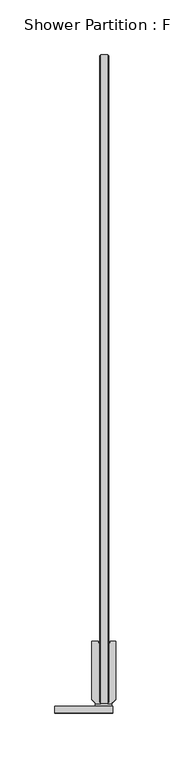
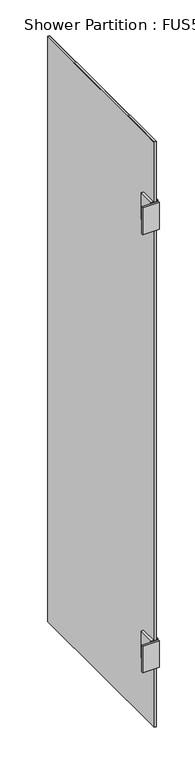
"""IFC4 building model written with IfcOpenShell, lengths in millimetres: furniture geometry, Shower Partition : FUS501_Shower Partition."""

import ifcopenshell
import ifcopenshell.guid

model = None  # the IFC model being written
_history = None  # IfcOwnerHistory: only IFC2X3 demands one
_inside = {}  # id of a spatial element -> (the spatial element, [elements in it])
_under = {}  # id of a project, library or spatial element -> (it, [spatial elements below it])
_declared = {}  # id of a project -> (the project, [libraries it declares])
_typed = {}  # id of a type object -> (the type object, [elements of that type])
_made_of = {}  # id of a material, layer set ... -> (it, [elements and type objects made of it])


def new_model(schema):
    """Start an empty IFC model of exactly this schema.

    Asked for "IFC4X3", IfcOpenShell would pick the latest addendum, in which some entities
    have other attributes; the version numbers below select the first issue.
    IFC2X3 requires an IfcOwnerHistory on every rooted entity: one is made here for all.
    """
    global model, _history
    if schema == "IFC4X3":
        model = ifcopenshell.file(schema_version=(4, 3, 0, 0))
    else:
        model = ifcopenshell.file(schema=schema)
    _inside.clear()
    _under.clear()
    _declared.clear()
    _typed.clear()
    _made_of.clear()
    _history = None
    if model.schema == "IFC2X3":
        org = make("IfcOrganization", Name="unknown")
        user = make(
            "IfcPersonAndOrganization",
            ThePerson=make("IfcPerson", FamilyName="unknown"),
            TheOrganization=org,
        )
        app = make(
            "IfcApplication",
            ApplicationDeveloper=org,
            Version="unknown",
            ApplicationFullName="unknown",
            ApplicationIdentifier="unknown",
        )
        _history = make(
            "IfcOwnerHistory",
            OwningUser=user,
            OwningApplication=app,
            ChangeAction="ADDED",
            CreationDate=0,
        )
    return model


def make(cls, **values):
    """One entity of the class cls with the attributes given. An attribute that is None is left unset."""
    return model.create_entity(
        cls, **{name: value for name, value in values.items() if value is not None}
    )


def rooted(cls, **values):
    """An entity with a GlobalId (a new one), such as an element, a storey or a relation."""
    return make(cls, GlobalId=ifcopenshell.guid.new(), OwnerHistory=_history, **values)


def si_unit(unit_type, name, prefix=None):
    """IfcSIUnit, for example si_unit("LENGTHUNIT", "METRE", prefix="MILLI")."""
    return make("IfcSIUnit", UnitType=unit_type, Prefix=prefix, Name=name)


def assignment(units):
    """IfcUnitAssignment: the units of a project."""
    return None if units is None else make("IfcUnitAssignment", Units=units)


def point(xyz):
    """IfcCartesianPoint."""
    return None if xyz is None else make("IfcCartesianPoint", Coordinates=xyz)


def direction(xyz):
    """IfcDirection."""
    return None if xyz is None else make("IfcDirection", DirectionRatios=xyz)


def frame(location, z_axis=None, x_axis=None):
    """IfcAxis2Placement3D, a coordinate frame: its origin and axes. An axis left out is left unset."""
    return make(
        "IfcAxis2Placement3D",
        Location=point(location),
        Axis=direction(z_axis),
        RefDirection=direction(x_axis),
    )


def origin():
    """The frame at (0, 0, 0) with its axes left unset."""
    return frame((0.0, 0.0, 0.0))


def place(relative_to, where):
    """IfcLocalPlacement: puts the frame where relative to a parent placement (None: the world)."""
    return make(
        "IfcLocalPlacement", PlacementRelTo=relative_to, RelativePlacement=where
    )


def context(
    kind, dimensions, precision=None, world=None, true_north=None, identifier=None
):
    """IfcGeometricRepresentationContext, for example the 3D "Model" context."""
    return make(
        "IfcGeometricRepresentationContext",
        ContextIdentifier=identifier,
        ContextType=kind,
        CoordinateSpaceDimension=dimensions,
        Precision=precision,
        WorldCoordinateSystem=world,
        TrueNorth=true_north,
    )


def project(units=None, contexts=None):
    """IfcProject with its units and contexts."""
    return rooted(
        "IfcProject",
        Name="project",
        RepresentationContexts=contexts,
        UnitsInContext=assignment(units),
    )


def spatial(cls, under=None, at=None, **own):
    """A site, building, storey or space (cls), placed at a placement, below another one or the project."""
    s = rooted(cls, ObjectPlacement=at, **own)
    if under is not None:
        _under.setdefault(under.id(), (under, []))[1].append(s)
    return s


def faces_of(points, faces, orient=None, outer=None):
    """IfcFace entities. A face is a list of loops; a loop is a list of indices into points, from 0.

    orient and outer hold one flag for each loop. By default every Orientation is true, the
    first loop of a face is its IfcFaceOuterBound and the others are IfcFaceBound.
    """
    made = []
    for i, loops in enumerate(faces):
        bounds = []
        for j, loop in enumerate(loops):
            is_outer = j == 0 if outer is None else outer[i][j]
            bounds.append(
                make(
                    "IfcFaceOuterBound" if is_outer else "IfcFaceBound",
                    Bound=make("IfcPolyLoop", Polygon=[points[k] for k in loop]),
                    Orientation=True if orient is None else orient[i][j],
                )
            )
        made.append(make("IfcFace", Bounds=bounds))
    return made


def faceted_brep(points, faces, orient=None, outer=None, voids=None):
    """IfcFacetedBrep: a solid bounded by flat faces; with voids (closed shells), ...WithVoids."""
    shared = [point(p) for p in points]
    hull = make("IfcClosedShell", CfsFaces=faces_of(shared, faces, orient, outer))
    if voids is None:
        return make("IfcFacetedBrep", Outer=hull)
    return make(
        "IfcFacetedBrepWithVoids",
        Outer=hull,
        Voids=[
            make(cls, CfsFaces=faces_of(shared, fs, o, b)) for cls, fs, o, b in voids
        ],
    )


def shape(context_of_items, identifier, shape_type, items):
    """IfcShapeRepresentation: the items that make up one representation, for example the "Body"."""
    return make(
        "IfcShapeRepresentation",
        ContextOfItems=context_of_items,
        RepresentationIdentifier=identifier,
        RepresentationType=shape_type,
        Items=items,
    )


def source(mapping_origin, context_of_items, identifier, shape_type, items):
    """IfcRepresentationMap: a shape defined once, which mapped items show again and again."""
    return make(
        "IfcRepresentationMap",
        MappingOrigin=mapping_origin,
        MappedRepresentation=shape(context_of_items, identifier, shape_type, items),
    )


def transform(
    local_origin,
    x_axis=None,
    y_axis=None,
    z_axis=None,
    scale=None,
    scale2=None,
    scale3=None,
    uniform=True,
):
    """IfcCartesianTransformationOperator3D, or its non-uniform kind. x_axis, y_axis, z_axis: its Axis1, 2, 3."""
    if uniform:
        return make(
            "IfcCartesianTransformationOperator3D",
            Axis1=direction(x_axis),
            Axis2=direction(y_axis),
            LocalOrigin=point(local_origin),
            Scale=scale,
            Axis3=direction(z_axis),
        )
    return make(
        "IfcCartesianTransformationOperator3DnonUniform",
        Axis1=direction(x_axis),
        Axis2=direction(y_axis),
        LocalOrigin=point(local_origin),
        Scale=scale,
        Axis3=direction(z_axis),
        Scale2=scale2,
        Scale3=scale3,
    )


def mapped(mapping_source, mapping_target):
    """IfcMappedItem: shows the shape of a source again, moved by a transform."""
    return make(
        "IfcMappedItem", MappingSource=mapping_source, MappingTarget=mapping_target
    )


def made_of(thing, what):
    """Note that an element or type object is made of a material, layer set ...; save() writes the relation."""
    if what is not None:
        _made_of.setdefault(what.id(), (what, []))[1].append(thing)
    return thing


def element(
    cls,
    number,
    at=None,
    inside=None,
    cuts=None,
    type_object=None,
    material=None,
    context=None,
    identifier="Body",
    shape_type=None,
    held_by="IfcProductDefinitionShape",
    body=None,
    shapes=None,
    **own,
):
    """One element of the class cls, such as IfcWall. Its Tag is "e" and its number.

    at: its placement. inside: the storey or other place that contains it. cuts: it is an
    opening in that element (IfcRelVoidsElement). A single representation is given by context,
    identifier, shape_type and body (its items); several are given by shapes. held_by: the class
    of the entity that holds the representations. save() writes the other relations.
    """
    e = rooted(cls, Tag="e%d" % number, ObjectPlacement=at, **own)
    if body is not None:
        shapes = [shape(context, identifier, shape_type, body)]
    if shapes is not None:
        e.Representation = make(held_by, Representations=shapes)
    if inside is not None:
        _inside.setdefault(inside.id(), (inside, []))[1].append(e)
    if cuts is not None:
        rooted(
            "IfcRelVoidsElement", RelatingBuildingElement=cuts, RelatedOpeningElement=e
        )
    if type_object is not None:
        _typed.setdefault(type_object.id(), (type_object, []))[1].append(e)
    return made_of(e, material)


def aggregate(whole, parts):
    """IfcRelAggregates: a whole, such as a stair, and the parts it consists of."""
    return rooted("IfcRelAggregates", RelatingObject=whole, RelatedObjects=parts)


def save(model, path):
    """Write the relations noted so far, then the file.

    IfcRelAggregates (storeys below a building ...), IfcRelContainedInSpatialStructure (elements
    in a storey), IfcRelDefinesByType, IfcRelAssociatesMaterial and IfcRelDeclares: one each for
    every whole, place, type object, material and project.
    """
    for whole, parts in _under.values():
        aggregate(whole, parts)
    for where, things in _inside.values():
        rooted(
            "IfcRelContainedInSpatialStructure",
            RelatedElements=things,
            RelatingStructure=where,
        )
    for kind, things in _typed.values():
        rooted("IfcRelDefinesByType", RelatedObjects=things, RelatingType=kind)
    for what, things in _made_of.values():
        rooted("IfcRelAssociatesMaterial", RelatedObjects=things, RelatingMaterial=what)
    for by, libraries in _declared.values():
        rooted("IfcRelDeclares", RelatingContext=by, RelatedDefinitions=libraries)
    model.write(path)


def shower_partition_fus501_shower_partition_aa17ee34(model_context):
    return source(origin(), model_context, "Body", "Brep", [
        faceted_brep([(17.0, -294.0, 1761.208438), (17.0, -291.5, 1761.208438), (13.0420514, -291.5, 1761.208438), (6.9579486, -291.5, 1761.208438), (2.0, -291.5, 1761.208438), (2.0, -294.0, 1761.208438), (17.0, -291.5, 1785.5), (13.0420514, -291.5, 1785.5), (6.9579486, -291.5, 1785.5), (2.0, -291.5, 1785.5), (2.0, -291.5, 1713.920216), (2.0, -291.5, 1694.5), (6.9579486, -291.5, 1694.5), (6.9579486, -291.5, 1713.920216), (13.0420514, -291.5, 1713.920216), (13.0420514, -291.5, 1694.5), (17.0, -291.5, 1694.5), (17.0, -291.5, 1713.920216), (2.0, -294.0, 1713.920216), (17.0, -294.0, 1713.920216), (2.0, -290.5420514, 1785.5), (6.0, -290.5420514, 1785.5), (6.0, -236.5, 1785.5), (4.5, -236.5, 1785.5), (4.5, -234.5, 1785.5), (-1.5, -234.5, 1785.5), (-1.5, -287.828945, 1785.5), (1.2131065, -290.5420514, 1785.5), (17.0, -290.5420514, 1785.5), (17.7868935, -290.5420514, 1785.5), (20.5, -287.828945, 1785.5), (20.5, -234.5, 1785.5), (15.5, -234.5, 1785.5), (15.5, -236.5, 1785.5), (14.0, -236.5, 1785.5), (14.0, -290.5420514, 1785.5), (-35.0, -294.0, 1785.5), (-35.0, -300.0, 1785.5), (17.8567847, -300.0, 1785.5), (17.8567847, -294.0, 1785.5), (17.0, -290.5420514, 1694.5), (14.0, -290.5420514, 1694.5), (14.0, -236.5, 1694.5), (15.5, -236.5, 1694.5), (15.5, -234.5, 1694.5), (20.5, -234.5, 1694.5), (20.5, -287.828945, 1694.5), (17.7868935, -290.5420514, 1694.5), (2.0, -290.5420514, 1694.5), (1.2131065, -290.5420514, 1694.5), (-1.5, -287.828945, 1694.5), (-1.5, -234.5, 1694.5), (4.5, -234.5, 1694.5), (4.5, -236.5, 1694.5), (6.0, -236.5, 1694.5), (6.0, -290.5420514, 1694.5), (17.8567847, -294.0, 1694.5), (17.8567847, -300.0, 1694.5), (-35.0, -300.0, 1694.5), (-35.0, -294.0, 1694.5)], [[[0, 1, 2, 3, 4, 5]], [[1, 6, 7, 2]], [[3, 8, 9, 4]], [[10, 11, 12, 13]], [[14, 15, 16, 17]], [[18, 10, 13, 14, 17, 19]], [[20, 9, 8, 21, 22, 23, 24, 25, 26, 27]], [[7, 6, 28, 29, 30, 31, 32, 33, 34, 35]], [[36, 37, 38, 39]], [[40, 16, 15, 41, 42, 43, 44, 45, 46, 47]], [[12, 11, 48, 49, 50, 51, 52, 53, 54, 55]], [[56, 57, 58, 59]], [[36, 39, 56, 59], [5, 18, 19, 0]], [[48, 11, 10, 18, 5, 4, 9, 20]], [[27, 49, 48, 20]], [[26, 50, 49, 27]], [[25, 51, 50, 26]], [[24, 52, 51, 25]], [[23, 53, 52, 24]], [[34, 42, 41, 35]], [[33, 43, 42, 34]], [[32, 44, 43, 33]], [[31, 45, 44, 32]], [[30, 46, 45, 31]], [[29, 47, 46, 30]], [[28, 40, 47, 29]], [[28, 6, 1, 0, 19, 17, 16, 40]], [[38, 57, 56, 39]], [[37, 58, 57, 38]], [[36, 59, 58, 37]], [[22, 54, 53, 23]], [[21, 55, 54, 22]], [[8, 3, 13, 12, 55, 21]], [[3, 2, 14, 13]], [[35, 41, 15, 14, 2, 7]]]),
        faceted_brep([(2.0, -290.5420514, 295.5), (2.0, -291.5, 295.5), (6.9579486, -291.5, 295.5), (6.0, -290.5420514, 295.5), (6.0, -236.5, 295.5), (4.5, -236.5, 295.5), (4.5, -234.5, 295.5), (-1.5, -234.5, 295.5), (-1.5, -287.828945, 295.5), (1.2131065, -290.5420514, 295.5), (13.0420514, -291.5, 295.5), (17.0, -291.5, 295.5), (17.0, -290.5420514, 295.5), (17.7868935, -290.5420514, 295.5), (20.5, -287.828945, 295.5), (20.5, -234.5, 295.5), (15.5, -234.5, 295.5), (15.5, -236.5, 295.5), (14.0, -236.5, 295.5), (14.0, -290.5420514, 295.5), (-35.0, -294.0, 295.5), (-35.0, -300.0, 295.5), (17.8567847, -300.0, 295.5), (17.8567847, -294.0, 295.5), (17.0, -290.5420514, 204.5), (17.0, -291.5, 204.5), (13.0420514, -291.5, 204.5), (14.0, -290.5420514, 204.5), (14.0, -236.5, 204.5), (15.5, -236.5, 204.5), (15.5, -234.5, 204.5), (20.5, -234.5, 204.5), (20.5, -287.828945, 204.5), (17.7868935, -290.5420514, 204.5), (6.9579486, -291.5, 204.5), (2.0, -291.5, 204.5), (2.0, -290.5420514, 204.5), (1.2131065, -290.5420514, 204.5), (-1.5, -287.828945, 204.5), (-1.5, -234.5, 204.5), (4.5, -234.5, 204.5), (4.5, -236.5, 204.5), (6.0, -236.5, 204.5), (6.0, -290.5420514, 204.5), (17.8567847, -294.0, 204.5), (17.8567847, -300.0, 204.5), (-35.0, -300.0, 204.5), (-35.0, -294.0, 204.5), (2.0, -294.0, 276.079784), (2.0, -294.0, 226.670216), (17.0, -294.0, 226.670216), (17.0, -294.0, 276.079784), (2.0, -291.5, 226.670216), (2.0, -291.5, 276.079784), (17.0, -291.5, 276.079784), (17.0, -291.5, 226.670216), (13.0420514, -291.5, 276.079784), (6.9579486, -291.5, 276.079784), (6.9579486, -291.5, 226.670216), (13.0420514, -291.5, 226.670216)], [[[0, 1, 2, 3, 4, 5, 6, 7, 8, 9]], [[10, 11, 12, 13, 14, 15, 16, 17, 18, 19]], [[20, 21, 22, 23]], [[24, 25, 26, 27, 28, 29, 30, 31, 32, 33]], [[34, 35, 36, 37, 38, 39, 40, 41, 42, 43]], [[44, 45, 46, 47]], [[20, 23, 44, 47], [48, 49, 50, 51]], [[36, 35, 52, 49, 48, 53, 1, 0]], [[9, 37, 36, 0]], [[8, 38, 37, 9]], [[7, 39, 38, 8]], [[6, 40, 39, 7]], [[5, 41, 40, 6]], [[18, 28, 27, 19]], [[17, 29, 28, 18]], [[16, 30, 29, 17]], [[15, 31, 30, 16]], [[14, 32, 31, 15]], [[13, 33, 32, 14]], [[12, 24, 33, 13]], [[12, 11, 54, 51, 50, 55, 25, 24]], [[22, 45, 44, 23]], [[21, 46, 45, 22]], [[20, 47, 46, 21]], [[51, 54, 56, 57, 53, 48]], [[54, 11, 10, 56]], [[57, 2, 1, 53]], [[52, 35, 34, 58]], [[59, 26, 25, 55]], [[49, 52, 58, 59, 55, 50]], [[4, 42, 41, 5]], [[3, 43, 42, 4]], [[2, 57, 58, 34, 43, 3]], [[57, 56, 59, 58]], [[19, 27, 26, 59, 56, 10]]]),
        faceted_brep([(13.0420514, 300.0, 0.0), (13.0420514, -291.5, 0.0), (6.9579486, -291.5, 0.0), (6.9579486, 300.0, 0.0), (13.0420514, -291.5, 1990.0), (13.0420514, 300.0, 1990.0), (6.9579486, 300.0, 1990.0), (6.9579486, -291.5, 1990.0), (6.0, 299.0420514, 0.9579486), (6.0, -290.5420514, 0.9579486), (6.0, -290.5420514, 1989.0420514), (6.0, 299.0420514, 1989.0420514), (14.0, 299.0420514, 1989.0420514), (14.0, -290.5420514, 1989.0420514), (14.0, -290.5420514, 0.9579486), (14.0, 299.0420514, 0.9579486)], [[[0, 1, 2, 3]], [[4, 5, 6, 7]], [[3, 6, 5, 0]], [[8, 9, 10, 11]], [[1, 4, 7, 2]], [[12, 13, 14, 15]], [[8, 11, 6, 3]], [[3, 2, 9, 8]], [[2, 7, 10, 9]], [[11, 10, 7, 6]], [[0, 5, 12, 15]], [[15, 14, 1, 0]], [[14, 13, 4, 1]], [[5, 4, 13, 12]]]),
    ])


if __name__ == "__main__":
    model = new_model("IFC4")
    model_context = context("Model", 3, world=origin())
    ifc_project = project(units=[si_unit("LENGTHUNIT", "METRE", prefix="MILLI")], contexts=[model_context])
    site = spatial("IfcSite", under=ifc_project)
    building = spatial("IfcBuilding", under=site)
    placement = place(None, origin())
    shower_partition_fus501_shower_partition_shape = shower_partition_fus501_shower_partition_aa17ee34(model_context)
    element("IfcFurniture", 1, ObjectType="Shower Partition : FUS501_Shower Partition", at=placement, inside=building, context=model_context, shape_type="MappedRepresentation", body=[
        mapped(shower_partition_fus501_shower_partition_shape, transform((0.0, 0.0, 0.0), x_axis=(1.0, 0.0, 0.0), y_axis=(0.0, 1.0, 0.0), z_axis=(0.0, 0.0, 1.0))),
    ])
    save(model, "model.ifc")

# Revit data of these elements
# Type "Shower Partition : FUS501_Shower Partition"
#   Youtube clip = ""
#   Weight Net (Kg) = "0"
#   Weight = ""
#   WarrantyStartDate [instance default] = "n/a"
#   WarrantyGuarantorParts = "n/a"
#   WarrantyGuarantorLabor = "n/a"
#   WarrantyDurationUnit = "Year"
#   WarrantyDurationParts = "n/a"
#   WarrantyDurationLabor = "n/a"
#   WarrantyDescription = "n/a"
#   VersionDate = "03/02/2020"
#   Version = "1"
#   Uniformat II Description = ""
#   Uniformat II Code = ""
#   Uniclass2015Reference = "Pr_40_20_06_79"
#   Uniclass2015Description = "Shower enclosures"
#   Uniclass2 = "Pr_40_30_06_79"
#   Uniclass 2015 Name = ""
#   Uniclass 2015 Code = ""
#   Uniclass 2.0 Description = ""
#   Uniclass 2.0 Code = ""
#   Uniclass 1.4 Description = ""
#   Uniclass 1.4 Code = ""
#   URL = "https://www.svedbergs.com/products/showers/shower-screen/180-shower-screen-1-door-78-206348/"
#   UNSPSC Code = ""
#   Technical description = ""
#   TagNumber [instance default] = "n/a"
#   SustainabilityPerformance = "n/a"
#   Style = "n/a"
#   Size = "70x780x2000mm"
#   Shape = "Rectangular"
#   SerialNumber [instance default] = "n/a"
#   Revision = "n/a"
#   ReplacementCost = "n/a"
#   Region South America = "All"
#   Region Oceania = "All"
#   Region North America = "All"
#   Region Middle East = "All"
#   Region Europe = "All"
#   Region Asia = "All"
#   Region Antarctica = "All"
#   Region Africa = "All"
#   RSKNumber = "7331415"
#   QR code = "http://bimobject.com/svedbergs/product/shower-78_shower"
#   ProductInformation = "Has one opening door. Doors can be folded inwards when shower is not in use to maximise floor space. No threshold – allows disabled access. Toughened safety glass 8 mm. Self-closing hinges. Concealed mounting & clamping screws. Height 200 cm. Door opening 75-95 cm."
#   ProductDatasheet = "https://www.svedbergs.com/products/showers/shower-screen/180-shower-screen-1-door-78-206348/GetPdf/?code=206348&productName=180%C2%B0%20Shower%20screen%201%20door%2078"
#   Product url = "https://www.svedbergs.com/products/showers/shower-screen/180-shower-screen-1-door-78-206348/"
#   Product group = "Shower Screen"
#   Product family = "180"
#   Product data url = "https://bimobject.com/svedbergs/product/shower-78_shower"
#   Product certification = ""
#   Product SKU = "shower-78_shower"
#   Product Guid = "bad75198-8fba-4d63-8e5f-588e794387c3"
#   OmniClass Description = ""
#   OmniClass Code = ""
#   Name = "180_Shower-screen_78"
#   NBSReference = "45-35-70/332"
#   NBSDescription = "Shower enclosures"
#   NBS Reference Description = ""
#   NBS Reference Code = ""
#   ModelReference = "681778"
#   ModelNumber = "n/a"
#   Material secondary = ""
#   Material main = ""
#   Material = "Glass, metal"
#   Masterformat 2014 Description = ""
#   Masterformat 2014 Code = ""
#   ManufacturerURL = "https://www.svedbergs.com/"
#   ManufacturerName = "Svedbergs"
#   Manufacturer name = ""
#   Manufacturer country = "Sweden"
#   MainColor = "Transparent"
#   InstallationDate [instance default] = "n/a"
#   Installation instructions = ""
#   IFC Classification = ""
#   GTIN code = ""
#   EANNumber = "7323100206787"
#   Design country = "Sweden"
#   Description = "Has one opening door. Doors can be folded inwards when shower is not in use to maximise floor space. No threshold – allows disabled access. Toughened safety glass 8 mm. Self-closing hinges. Concealed mounting & clamping screws. Height 200 cm. Door opening 75-95 cm."
#   Date of publishing = ""
#   Collection = "180°"
#   Model = "180° Shower Door 78 - Chrome/Clear glass"
#   Manufacturer = "Svedbergs"
#   IfcExportType = "NOTDEFINED"
#   IfcExportAs = "IfcFurnitureType"
#   Grade = "n/a"
#   Finish = "Black Mat/Clear glass"
#   Features = "Accessories:Shower seat Relax"
#   ExpectedLife = "n/a"
#   DurationUnit = "Year"
#   ConvergoRefNr = "0056-1912-0096-SE\t\t\r\n"
#   Constituents = "n/a"
#   Color = "Transparent"
#   CodePerformance = "n/a"
#   Category = "Shower screen"
#   COBIe Type Category = ""
#   Brand url = "http://www.svedbergs.com/"
#   Brand = "Svedbergs"
#   Barcode [instance default] = "n/a"
#   BIMobject main category code = "sanitary"
#   BIMobject main category = "Sanitary"
#   BIMobject category code = "sanitary-shower-screens"
#   BIMobject category = "Shower screens"
#   BIMObjectName = "Sanitary_Shower-screens_Svedbergs_180_Shower-screen_78"
#   Author = "Convergo AB"
#   AssetType = "Fixed"
#   AssetIdentifier [instance default] = "n/a"
#   AssemblyInstruction = "https://www.svedbergs.com/globalassets/catalog-assets/documentfile/99248-M1_180_dorr.pdf"
#   AccessibilityPerformance = "n/a"
#   NominalLength = 70 mm
#   NominalDepth = 600 mm
#   Nominal width = 0 mm
#   Nominal height = 0 mm
#   Edition number = 1
#   ShowerEnclosureSecondaryMaterial = Black Mat
#   ShowerEnclosureMainMaterial = Clear Glass
#   Type Comments = ""
#   Default Elevation = 0
#   Cost = 0
# Element 1 (IfcFurniture, "Shower Partition : FUS501_Shower Partition")
#   Materials on its faces: "Black Mat", "Clear Glass"
# Materials
#   "Black Mat": class "Metal", colour RGB 20 20 20, transparency 0, Cost = 0
#   "Clear Glass": class "Glass", colour RGB 236 240 239, transparency 0.85, Description = "Clear glazing", Cost = 0
